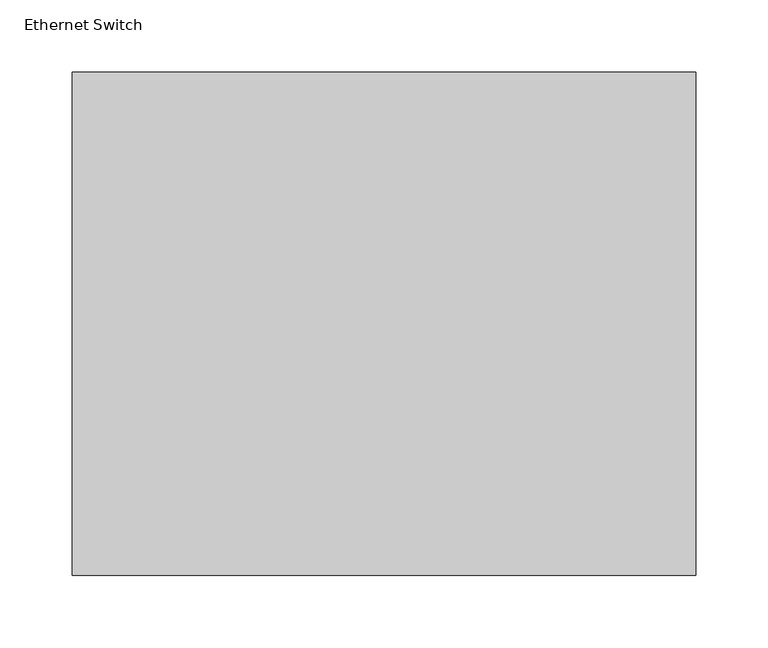
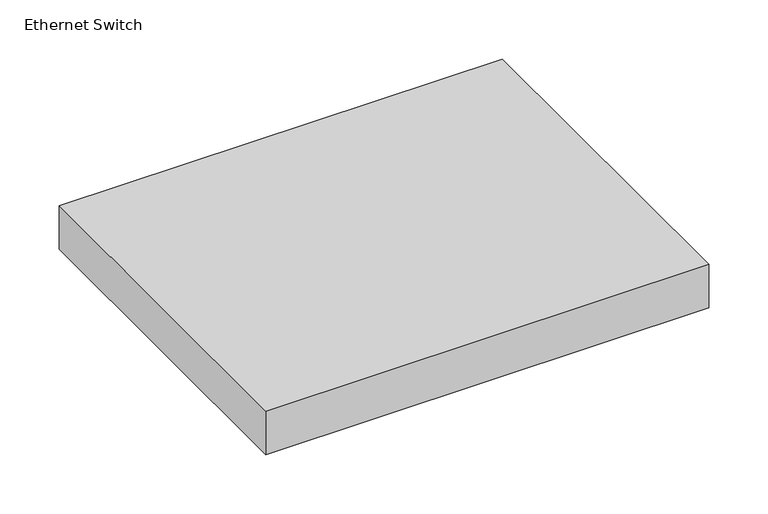
"""IFC4 building model written with IfcOpenShell, lengths in millimetres: proxy geometry, Ethernet Switch : NETGEAR 16 Port Gigabit Ethernet Plus Network Switch (GS116E)."""

import ifcopenshell
import ifcopenshell.guid

model = None  # the IFC model being written
_history = None  # IfcOwnerHistory: only IFC2X3 demands one
_inside = {}  # id of a spatial element -> (the spatial element, [elements in it])
_under = {}  # id of a project, library or spatial element -> (it, [spatial elements below it])
_declared = {}  # id of a project -> (the project, [libraries it declares])
_typed = {}  # id of a type object -> (the type object, [elements of that type])
_made_of = {}  # id of a material, layer set ... -> (it, [elements and type objects made of it])


def new_model(schema):
    """Start an empty IFC model of exactly this schema.

    Asked for "IFC4X3", IfcOpenShell would pick the latest addendum, in which some entities
    have other attributes; the version numbers below select the first issue.
    IFC2X3 requires an IfcOwnerHistory on every rooted entity: one is made here for all.
    """
    global model, _history
    if schema == "IFC4X3":
        model = ifcopenshell.file(schema_version=(4, 3, 0, 0))
    else:
        model = ifcopenshell.file(schema=schema)
    _inside.clear()
    _under.clear()
    _declared.clear()
    _typed.clear()
    _made_of.clear()
    _history = None
    if model.schema == "IFC2X3":
        org = make("IfcOrganization", Name="unknown")
        user = make(
            "IfcPersonAndOrganization",
            ThePerson=make("IfcPerson", FamilyName="unknown"),
            TheOrganization=org,
        )
        app = make(
            "IfcApplication",
            ApplicationDeveloper=org,
            Version="unknown",
            ApplicationFullName="unknown",
            ApplicationIdentifier="unknown",
        )
        _history = make(
            "IfcOwnerHistory",
            OwningUser=user,
            OwningApplication=app,
            ChangeAction="ADDED",
            CreationDate=0,
        )
    return model


def make(cls, **values):
    """One entity of the class cls with the attributes given. An attribute that is None is left unset."""
    return model.create_entity(
        cls, **{name: value for name, value in values.items() if value is not None}
    )


def rooted(cls, **values):
    """An entity with a GlobalId (a new one), such as an element, a storey or a relation."""
    return make(cls, GlobalId=ifcopenshell.guid.new(), OwnerHistory=_history, **values)


def si_unit(unit_type, name, prefix=None):
    """IfcSIUnit, for example si_unit("LENGTHUNIT", "METRE", prefix="MILLI")."""
    return make("IfcSIUnit", UnitType=unit_type, Prefix=prefix, Name=name)


def assignment(units):
    """IfcUnitAssignment: the units of a project."""
    return None if units is None else make("IfcUnitAssignment", Units=units)


def point(xyz):
    """IfcCartesianPoint."""
    return None if xyz is None else make("IfcCartesianPoint", Coordinates=xyz)


def direction(xyz):
    """IfcDirection."""
    return None if xyz is None else make("IfcDirection", DirectionRatios=xyz)


def frame(location, z_axis=None, x_axis=None):
    """IfcAxis2Placement3D, a coordinate frame: its origin and axes. An axis left out is left unset."""
    return make(
        "IfcAxis2Placement3D",
        Location=point(location),
        Axis=direction(z_axis),
        RefDirection=direction(x_axis),
    )


def origin():
    """The frame at (0, 0, 0) with its axes left unset."""
    return frame((0.0, 0.0, 0.0))


def origin_with_axes():
    """The frame at (0, 0, 0) with the z axis (0, 0, 1) and the x axis (1, 0, 0) written out."""
    return frame((0.0, 0.0, 0.0), z_axis=(0.0, 0.0, 1.0), x_axis=(1.0, 0.0, 0.0))


def place(relative_to, where):
    """IfcLocalPlacement: puts the frame where relative to a parent placement (None: the world)."""
    return make(
        "IfcLocalPlacement", PlacementRelTo=relative_to, RelativePlacement=where
    )


def context(
    kind, dimensions, precision=None, world=None, true_north=None, identifier=None
):
    """IfcGeometricRepresentationContext, for example the 3D "Model" context."""
    return make(
        "IfcGeometricRepresentationContext",
        ContextIdentifier=identifier,
        ContextType=kind,
        CoordinateSpaceDimension=dimensions,
        Precision=precision,
        WorldCoordinateSystem=world,
        TrueNorth=true_north,
    )


def project(units=None, contexts=None):
    """IfcProject with its units and contexts."""
    return rooted(
        "IfcProject",
        Name="project",
        RepresentationContexts=contexts,
        UnitsInContext=assignment(units),
    )


def spatial(cls, under=None, at=None, **own):
    """A site, building, storey or space (cls), placed at a placement, below another one or the project."""
    s = rooted(cls, ObjectPlacement=at, **own)
    if under is not None:
        _under.setdefault(under.id(), (under, []))[1].append(s)
    return s


def polyline(points):
    """IfcPolyline through the points."""
    return make("IfcPolyline", Points=[point(p) for p in points])


def outline(outer, holes=None, kind="AREA"):
    """IfcArbitraryClosedProfileDef: a profile drawn as a closed curve; with holes, ...WithVoids."""
    if holes is None:
        return make("IfcArbitraryClosedProfileDef", ProfileType=kind, OuterCurve=outer)
    return make(
        "IfcArbitraryProfileDefWithVoids",
        ProfileType=kind,
        OuterCurve=outer,
        InnerCurves=holes,
    )


def extrude(swept, where, along, depth):
    """IfcExtrudedAreaSolid: the profile swept, set in the frame where, extruded along a direction by depth."""
    return make(
        "IfcExtrudedAreaSolid",
        SweptArea=swept,
        Position=where,
        ExtrudedDirection=direction(along),
        Depth=depth,
    )


def shape(context_of_items, identifier, shape_type, items):
    """IfcShapeRepresentation: the items that make up one representation, for example the "Body"."""
    return make(
        "IfcShapeRepresentation",
        ContextOfItems=context_of_items,
        RepresentationIdentifier=identifier,
        RepresentationType=shape_type,
        Items=items,
    )


def source(mapping_origin, context_of_items, identifier, shape_type, items):
    """IfcRepresentationMap: a shape defined once, which mapped items show again and again."""
    return make(
        "IfcRepresentationMap",
        MappingOrigin=mapping_origin,
        MappedRepresentation=shape(context_of_items, identifier, shape_type, items),
    )


def transform(
    local_origin,
    x_axis=None,
    y_axis=None,
    z_axis=None,
    scale=None,
    scale2=None,
    scale3=None,
    uniform=True,
):
    """IfcCartesianTransformationOperator3D, or its non-uniform kind. x_axis, y_axis, z_axis: its Axis1, 2, 3."""
    if uniform:
        return make(
            "IfcCartesianTransformationOperator3D",
            Axis1=direction(x_axis),
            Axis2=direction(y_axis),
            LocalOrigin=point(local_origin),
            Scale=scale,
            Axis3=direction(z_axis),
        )
    return make(
        "IfcCartesianTransformationOperator3DnonUniform",
        Axis1=direction(x_axis),
        Axis2=direction(y_axis),
        LocalOrigin=point(local_origin),
        Scale=scale,
        Axis3=direction(z_axis),
        Scale2=scale2,
        Scale3=scale3,
    )


def mapped(mapping_source, mapping_target):
    """IfcMappedItem: shows the shape of a source again, moved by a transform."""
    return make(
        "IfcMappedItem", MappingSource=mapping_source, MappingTarget=mapping_target
    )


def made_of(thing, what):
    """Note that an element or type object is made of a material, layer set ...; save() writes the relation."""
    if what is not None:
        _made_of.setdefault(what.id(), (what, []))[1].append(thing)
    return thing


def element(
    cls,
    number,
    at=None,
    inside=None,
    cuts=None,
    type_object=None,
    material=None,
    context=None,
    identifier="Body",
    shape_type=None,
    held_by="IfcProductDefinitionShape",
    body=None,
    shapes=None,
    **own,
):
    """One element of the class cls, such as IfcWall. Its Tag is "e" and its number.

    at: its placement. inside: the storey or other place that contains it. cuts: it is an
    opening in that element (IfcRelVoidsElement). A single representation is given by context,
    identifier, shape_type and body (its items); several are given by shapes. held_by: the class
    of the entity that holds the representations. save() writes the other relations.
    """
    e = rooted(cls, Tag="e%d" % number, ObjectPlacement=at, **own)
    if body is not None:
        shapes = [shape(context, identifier, shape_type, body)]
    if shapes is not None:
        e.Representation = make(held_by, Representations=shapes)
    if inside is not None:
        _inside.setdefault(inside.id(), (inside, []))[1].append(e)
    if cuts is not None:
        rooted(
            "IfcRelVoidsElement", RelatingBuildingElement=cuts, RelatedOpeningElement=e
        )
    if type_object is not None:
        _typed.setdefault(type_object.id(), (type_object, []))[1].append(e)
    return made_of(e, material)


def aggregate(whole, parts):
    """IfcRelAggregates: a whole, such as a stair, and the parts it consists of."""
    return rooted("IfcRelAggregates", RelatingObject=whole, RelatedObjects=parts)


def save(model, path):
    """Write the relations noted so far, then the file.

    IfcRelAggregates (storeys below a building ...), IfcRelContainedInSpatialStructure (elements
    in a storey), IfcRelDefinesByType, IfcRelAssociatesMaterial and IfcRelDeclares: one each for
    every whole, place, type object, material and project.
    """
    for whole, parts in _under.values():
        aggregate(whole, parts)
    for where, things in _inside.values():
        rooted(
            "IfcRelContainedInSpatialStructure",
            RelatedElements=things,
            RelatingStructure=where,
        )
    for kind, things in _typed.values():
        rooted("IfcRelDefinesByType", RelatedObjects=things, RelatingType=kind)
    for what, things in _made_of.values():
        rooted("IfcRelAssociatesMaterial", RelatedObjects=things, RelatingMaterial=what)
    for by, libraries in _declared.values():
        rooted("IfcRelDeclares", RelatingContext=by, RelatedDefinitions=libraries)
    model.write(path)


def ethernet_switch_5c8040eb(model_context):
    return source(origin(), model_context, "Body", "SweptSolid", [
        extrude(outline(polyline([(216.05, 174.5), (216.05, -174.5), (-216.05, -174.5), (-216.05, 174.5), (216.05, 174.5)])), origin_with_axes(), (0.0, 0.0, 1.0), 44.9),
    ])


if __name__ == "__main__":
    model = new_model("IFC4")
    model_context = context("Model", 3, world=origin())
    ifc_project = project(units=[si_unit("LENGTHUNIT", "METRE", prefix="MILLI")], contexts=[model_context])
    site = spatial("IfcSite", under=ifc_project)
    building = spatial("IfcBuilding", under=site)
    placement = place(None, origin())
    ethernet_switch_shape = ethernet_switch_5c8040eb(model_context)
    element("IfcBuildingElementProxy", 1, Name="Ethernet Switch : NETGEAR 16 Port Gigabit Ethernet Plus Network Switch (GS116E)", ObjectType="Ethernet Switch : NETGEAR 16 Port Gigabit Ethernet Plus Network Switch (GS116E)", at=placement, inside=building, context=model_context, shape_type="MappedRepresentation", body=[
        mapped(ethernet_switch_shape, transform((0.0, 0.0, 0.0), x_axis=(1.0, 0.0, 0.0), y_axis=(0.0, 1.0, 0.0), z_axis=(0.0, 0.0, 1.0))),
    ])
    save(model, "model.ifc")

# Revit data of these elements
# Type "Ethernet Switch : NETGEAR 16 Port Gigabit Ethernet Plus Network Switch (GS116E)"
#   Width = 432.1 mm
#   Height = 44.9 mm
#   Depth = 349 mm
#   built-in parameter 1140087 [instance default] = 1
#   Default Elevation = 0
